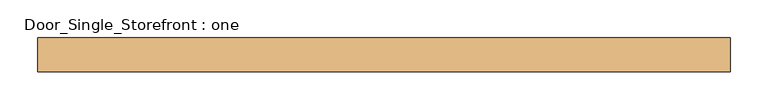
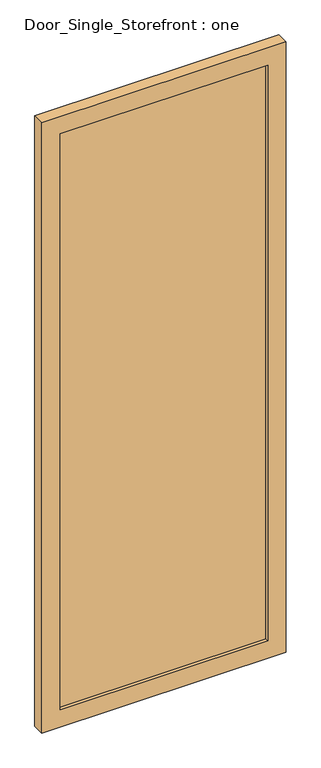
"""IFC4 building model written with IfcOpenShell, lengths in millimetres: door geometry, Door_Single_Storefront : one."""

from ifc_helpers import new_model, si_unit, frame, origin, place, context, project, spatial, polyline, outline, extrude, source, transform, mapped, element, save


def door_single_storefront_one_37df465a(model_context):
    return source(origin(), model_context, "Body", "SweptSolid", [
        extrude(outline(polyline([(388.9375, -6.35), (-388.9375, -6.35), (-388.9375, 12.7), (388.9375, 12.7), (388.9375, -6.35)])), frame((0.0, 0.0, 68.2625), z_axis=(0.0, 0.0, 1.0), x_axis=(1.0, 0.0, 0.0)), (0.0, 0.0, 1.0), 2276.2100966),
        extrude(outline(polyline([(2412.7350966, -457.2), (0.0, -457.2), (0.0, 457.2), (2412.7350966, 457.2), (2412.7350966, -457.2)]), holes=[polyline([(68.2625, 388.9375), (68.2625, -388.9375), (2344.4725966, -388.9375), (2344.4725966, 388.9375), (68.2625, 388.9375)])]), frame((0.0, -19.05, 0.0), z_axis=(0.0, 1.0, 0.0), x_axis=(0.0, 0.0, 1.0)), (0.0, 0.0, 1.0), 44.45),
    ])


if __name__ == "__main__":
    model = new_model("IFC4")
    model_context = context("Model", 3, world=origin())
    ifc_project = project(units=[si_unit("LENGTHUNIT", "METRE", prefix="MILLI")], contexts=[model_context])
    site = spatial("IfcSite", under=ifc_project)
    building = spatial("IfcBuilding", under=site)
    placement = place(None, origin())
    door_single_storefront_one_shape = door_single_storefront_one_37df465a(model_context)
    element("IfcDoor", 1, ObjectType="Door_Single_Storefront : one", at=placement, inside=building, context=model_context, shape_type="MappedRepresentation", body=[
        mapped(door_single_storefront_one_shape, transform((0.0, 0.0, 0.0), x_axis=(1.0, 0.0, 0.0), y_axis=(0.0, 1.0, 0.0), z_axis=(0.0, 0.0, 1.0))),
    ])
    save(model, "model.ifc")

# Revit data of these elements
# Type "Door_Single_Storefront : one"
#   Type Mark = "29"
#   OD_DS_Door_Material = "ALUM./GLAZING"
#   OD_DS_Door_Type = "STOREFRONT (NARROW STILE)"
#   OD_DS_Lockset = "ENTRY LOCK (INSIDE ADA LEVER ALWAYS ACTIVE)"
#   Analytic Construction = "<None>"
#   angle open [instance default] = 132.952°
#   Stile_Width = 0' - 2 11/16"
#   Door_Thickness = 0' - 1 3/4"
#   Door_Offset = 0' - 1"
#   Glass_Material = TEMPERED INSULATED GLAZING (CARDINAL GLASS LoĒ²-240\nOR EQUIVALENT)
#   Frame_Material = KAWNEER 260 INSULCLADTM THERMAL ENTRANCE - CLEAR ANODIZED ALUM.
#   Function = (empty or 0)
# Element 1 (IfcDoor, "Door_Single_Storefront : one")
#   Materials on its faces: "KAWNEER 260 INSULCLADTM THERMAL ENTRANCE - CLEAR ANODIZED ALUM.", "TEMPERED INSULATED GLAZING (CARDINAL GLASS LoĒ²-240\nOR EQUIVALENT)"
# Materials
#   "TEMPERED INSULATED GLAZING (CARDINAL GLASS LoĒ²-240\nOR EQUIVALENT)": class "Glass", colour RGB 196 205 210, transparency 0.85, Description = "Soda Lime Glass", Cost = 0
#   "KAWNEER 260 INSULCLADTM THERMAL ENTRANCE - CLEAR ANODIZED ALUM.": class "Metal", colour RGB 244 244 244, transparency 0, Description = "Aluminum 6061", Cost = 0
